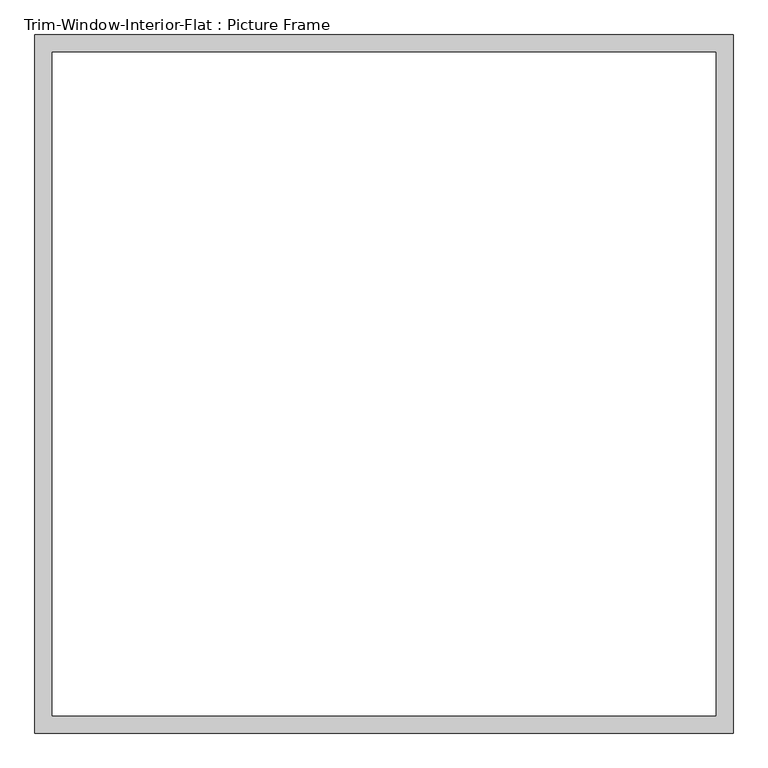
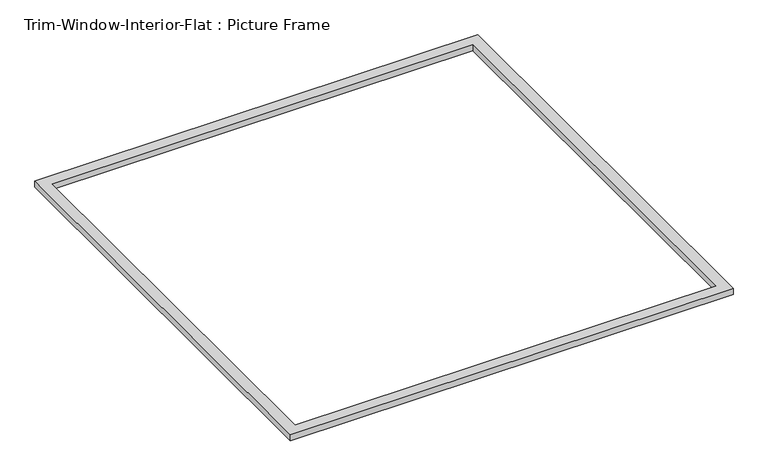
"""IFC4 building model written with IfcOpenShell, lengths in millimetres: proxy geometry, Trim-Window-Interior-Flat : Picture Frame."""

from ifc_helpers import new_model, si_unit, origin, origin_with_axes, place, context, project, spatial, polyline, outline, extrude, source, transform, mapped, element, save


def trim_window_interior_flat_picture_frame_0b66f2e0(model_context):
    return source(origin(), model_context, "Body", "SweptSolid", [
        extrude(outline(polyline([(1144.45, -44.45), (-1144.45, -44.45), (-1144.45, 2244.45), (1144.45, 2244.45), (1144.45, -44.45)]), holes=[polyline([(1087.3, 12.7), (1087.3, 2187.3), (-1087.3, 2187.3), (-1087.3, 12.7), (1087.3, 12.7)])]), origin_with_axes(), (0.0, 0.0, 1.0), 31.75),
    ])


if __name__ == "__main__":
    model = new_model("IFC4")
    model_context = context("Model", 3, world=origin())
    ifc_project = project(units=[si_unit("LENGTHUNIT", "METRE", prefix="MILLI")], contexts=[model_context])
    site = spatial("IfcSite", under=ifc_project)
    building = spatial("IfcBuilding", under=site)
    placement = place(None, origin())
    trim_window_interior_flat_picture_frame_shape = trim_window_interior_flat_picture_frame_0b66f2e0(model_context)
    element("IfcBuildingElementProxy", 1, Name="Trim-Window-Interior-Flat : Picture Frame", ObjectType="Trim-Window-Interior-Flat : Picture Frame", at=placement, inside=building, context=model_context, shape_type="MappedRepresentation", body=[
        mapped(trim_window_interior_flat_picture_frame_shape, transform((0.0, 0.0, 0.0), x_axis=(1.0, 0.0, 0.0), y_axis=(0.0, 1.0, 0.0), z_axis=(0.0, 0.0, 1.0))),
    ])
    save(model, "model.ifc")

# Revit data of these elements
# Type "Trim-Window-Interior-Flat : Picture Frame"
#   Trim Thickness_Picture Frame = 0.03175 m
#   Trim Width = 0.05715 m
#   Trim Thickness_with Sill = 0.01905 m
#   Sill Thickness = 0.03175 m
#   Opening Width [instance default] = 0.6096 m
#   Opening Height [instance default] = 0.9144 m
#   Default Elevation = 1.2192 m
#   Sill = no
#   Picture Frame = yes
#   Trim Material [instance default] = none
# Element 1 (IfcBuildingElementProxy, "Trim-Window-Interior-Flat : Picture Frame")
#   Opening Width = 2.2 m
#   Opening Height = 2.2 m
#   Trim Material = Wood - Stained
#   Materials on its faces: "Wood - Stained"
# Materials
#   "Wood - Stained": class "Wood", colour RGB 227 170 128, transparency 0, Cost = 0
